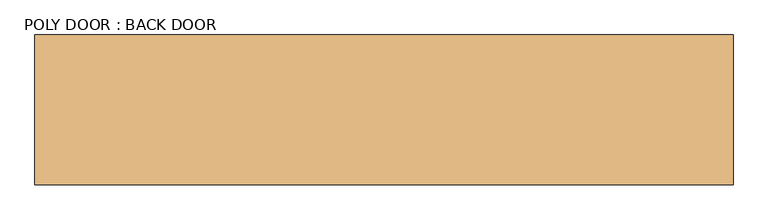
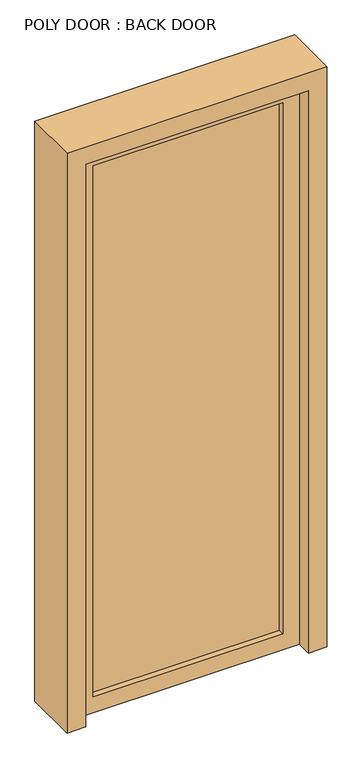
"""IFC4 building model written with IfcOpenShell, lengths in millimetres: door geometry, POLY DOOR : BACK DOOR."""

from ifc_helpers import new_model, si_unit, frame, origin, place, context, project, spatial, polyline, outline, extrude, source, transform, mapped, element, save


def poly_door_back_door_ba261477(model_context):
    return source(origin(), model_context, "Body", "SweptSolid", [
        extrude(outline(polyline([(388.9375, -25.4), (-388.9375, -25.4), (-388.9375, -12.7), (388.9375, -12.7), (388.9375, -25.4)])), frame((0.0, 0.0, 68.2625), z_axis=(0.0, 0.0, 1.0), x_axis=(1.0, 0.0, 0.0)), (0.0, 0.0, 1.0), 2301.875),
        extrude(outline(polyline([(2438.4, 457.2), (2438.4, -457.2), (0.0, -457.2), (0.0, 457.2), (2438.4, 457.2)]), holes=[polyline([(2370.1375, 388.9375), (68.2625, 388.9375), (68.2625, -388.9375), (2370.1375, -388.9375), (2370.1375, 388.9375)])]), frame((0.0, -50.8, 0.0), z_axis=(0.0, 1.0, 0.0), x_axis=(0.0, 0.0, 1.0)), (0.0, 0.0, 1.0), 50.8),
        extrude(outline(polyline([(2514.6, -533.4), (0.0, -533.4), (0.0, -457.2), (2438.4, -457.2), (2438.4, 457.2), (0.0, 457.2), (0.0, 533.4), (2514.6, 533.4), (2514.6, -533.4)])), frame((0.0, -114.3, 0.0), z_axis=(0.0, 1.0, 0.0), x_axis=(0.0, 0.0, 1.0)), (0.0, 0.0, 1.0), 228.6),
    ])


if __name__ == "__main__":
    model = new_model("IFC4")
    model_context = context("Model", 3, world=origin())
    ifc_project = project(units=[si_unit("LENGTHUNIT", "METRE", prefix="MILLI")], contexts=[model_context])
    site = spatial("IfcSite", under=ifc_project)
    building = spatial("IfcBuilding", under=site)
    placement = place(None, origin())
    poly_door_back_door_shape = poly_door_back_door_ba261477(model_context)
    element("IfcDoor", 1, ObjectType="POLY DOOR : BACK DOOR", at=placement, inside=building, context=model_context, shape_type="MappedRepresentation", body=[
        mapped(poly_door_back_door_shape, transform((0.0, 0.0, 0.0), x_axis=(1.0, 0.0, 0.0), y_axis=(0.0, 1.0, 0.0), z_axis=(0.0, 0.0, 1.0))),
    ])
    save(model, "model.ifc")

# Revit data of these elements
# Type "POLY DOOR : BACK DOOR"
#   Type Mark = "64"
#   OD_DS_Door_Material = "ALUM./GLAZING"
#   OD_DS_Door_Type = "STOREFRONT (NARROW STILE)"
#   OD_DS_Lockset = "ENTRY LOCK (INSIDE ADA LEVER ALWAYS ACTIVE)"
#   Assembly Code = "C1020"
#   Analytic Construction = "<None>"
#   Thickness = 0' - 2"
#   Glass Inset = 0' - 2 11/16"
#   Height = 8' - 0"
#   Trim Projection Ext = 0' - 1"
#   Trim Projection Int = 0' - 1"
#   Trim Width = 0' - 3"
#   Width = 3' - 0"
#   WINDOW = yes
#   Glass Material = TEMPERED INSULATED GLAZING (CARDINAL GLASS LoĒ²-240\nOR EQUIVALENT)
#   Door Material = KAWNEER 260 INSULCLADTM THERMAL ENTRANCE - CLEAR ANODIZED ALUM.
#   Frame Material = KAWNEER TRIFAB VERSAGLAZE 451T - CLEAR ANODIZED ALUM. - BACK GLAZED
#   Function = (empty or 0)
#   Wall Closure = (empty or 0)
# Element 1 (IfcDoor, "POLY DOOR : BACK DOOR")
#   Materials on its faces: "KAWNEER 260 INSULCLADTM THERMAL ENTRANCE - CLEAR ANODIZED ALUM.", "KAWNEER TRIFAB VERSAGLAZE 451T - CLEAR ANODIZED ALUM. - BACK GLAZED", "TEMPERED INSULATED GLAZING (CARDINAL GLASS LoĒ²-240\nOR EQUIVALENT)"
# Materials
#   "TEMPERED INSULATED GLAZING (CARDINAL GLASS LoĒ²-240\nOR EQUIVALENT)": class "Glass", colour RGB 196 205 210, transparency 0.85, Description = "Soda Lime Glass", Cost = 0
#   "KAWNEER 260 INSULCLADTM THERMAL ENTRANCE - CLEAR ANODIZED ALUM.": class "Metal", colour RGB 244 244 244, transparency 0, Description = "Aluminum 6061", Cost = 0
#   "KAWNEER TRIFAB VERSAGLAZE 451T - CLEAR ANODIZED ALUM. - BACK GLAZED": class "Metal", colour RGB 244 244 244, transparency 0, Description = "Aluminum 6061", Cost = 0
